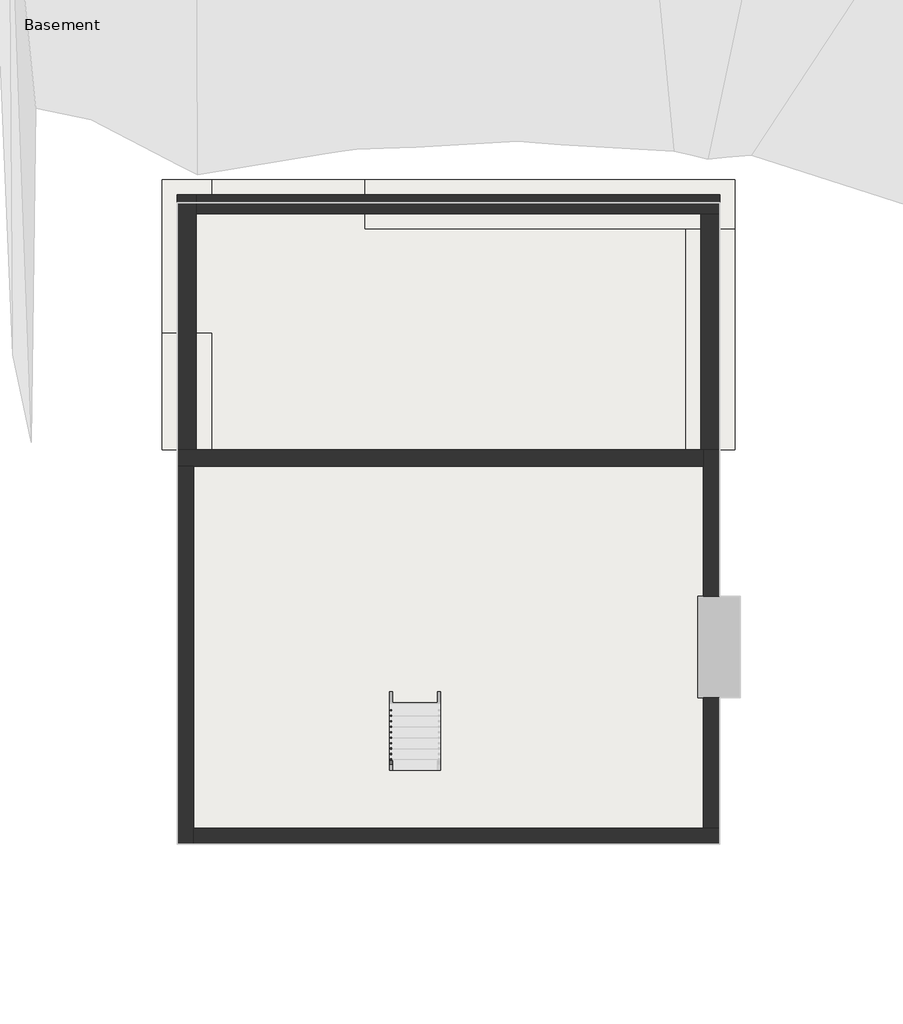
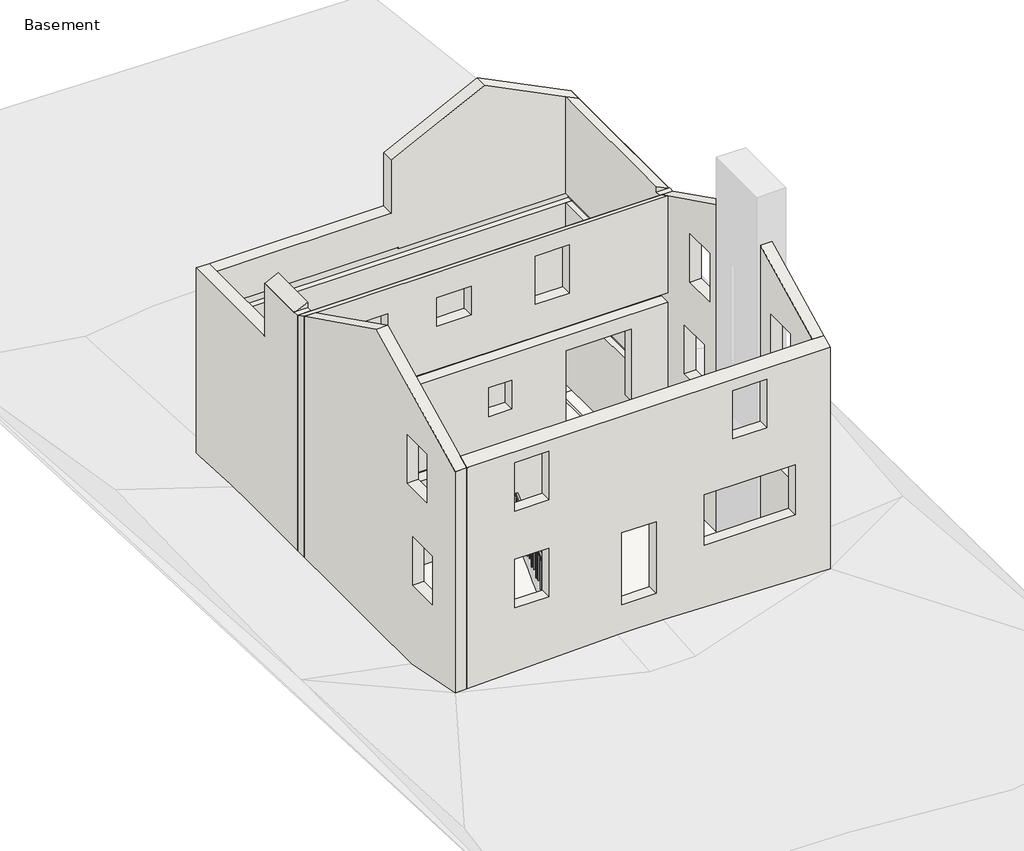
# One storey, part 1 of 2: 8 walls, 3 footings, 2 slabs, 1 railing.
"""IFC4 building model written with IfcOpenShell, lengths in millimetres."""

from ifc_helpers import new_model, si_unit, frame, origin, place, context, project, spatial, polyline, outline, extrude, faceted_brep, element, save

model = new_model("IFC4")

# Units and contexts
model_context = context("Model", 3, world=origin())
ifc_project = project(units=[si_unit("LENGTHUNIT", "METRE", prefix="MILLI")], contexts=[model_context])

# Site, building, storey
site = spatial("IfcSite", under=ifc_project)
building = spatial("IfcBuilding", under=site)
storey = spatial("IfcBuildingStorey", under=building, Name="Basement", Elevation=-2667.0)

# Footings
placement = place(None, origin())
element("IfcFooting", 1, ObjectType="Bearing Footing - 36\" x 12\"", at=placement, inside=storey, context=model_context, shape_type="Brep", body=[
    faceted_brep([(-5355.7678068, 3152.0888758, -2667.0), (-6270.1678068, 3152.0888758, -2667.0), (-6270.1678068, 3152.0888758, -2971.8), (-5355.7678068, 3152.0888758, -2971.8), (-6270.1678068, 5311.0888758, -2667.0), (-5355.7678068, 5311.0888758, -2667.0), (-5355.7678068, 5311.0888758, -2971.8), (-6270.1678068, 5311.0888758, -2971.8)], [[[0, 1, 2, 3]], [[4, 5, 6, 7]], [[0, 5, 4, 1]], [[2, 1, 4, 7]], [[3, 2, 7, 6]], [[0, 3, 6, 5]]]),
    faceted_brep([(-5355.7678068, 5311.0888758, -3124.2), (-6270.1678068, 5311.0888758, -3124.2), (-6270.1678068, 5311.0888758, -3429.0), (-5355.7678068, 5311.0888758, -3429.0), (-5355.7678068, 7243.0763758, -3124.2), (-5355.7678068, 8157.4763758, -3124.2), (-6270.1678068, 8157.4763758, -3124.2), (-6270.1678068, 8157.4763758, -3429.0), (-5355.7678068, 8157.4763758, -3429.0), (-5355.7678068, 7243.0763758, -3429.0)], [[[0, 1, 2, 3]], [[0, 4, 5, 6, 1]], [[2, 1, 6, 7]], [[3, 2, 7, 8, 9]], [[0, 3, 9, 8, 5, 4]], [[6, 5, 8, 7]]]),
])
element("IfcFooting", 2, ObjectType="Bearing Footing - 36\" x 12\"", at=placement, inside=storey, context=model_context, shape_type="Brep", body=[
    faceted_brep([(-2509.3803068, 8157.4763758, -3429.0), (-2509.3803068, 8157.4763758, -3124.2), (-2509.3803068, 7243.0763758, -3124.2), (-2509.3803068, 7243.0763758, -3429.0), (-5355.7678068, 8157.4763758, -3124.2), (-5355.7678068, 7243.0763758, -3124.2), (-5355.7678068, 8157.4763758, -3429.0), (-5355.7678068, 7243.0763758, -3429.0)], [[[0, 1, 2, 3]], [[2, 1, 4, 5]], [[1, 0, 6, 4]], [[0, 3, 7, 6]], [[3, 2, 5, 7]], [[5, 4, 6, 7]]]),
    faceted_brep([(-2509.3803068, 8157.4763758, -2667.0), (-2509.3803068, 8157.4763758, -2971.8), (-2509.3803068, 7243.0763758, -2971.8), (-2509.3803068, 7243.0763758, -2667.0), (4350.2071932, 8157.4763758, -2667.0), (3435.8071932, 7243.0763758, -2667.0), (4350.2071932, 7243.0763758, -2667.0), (4350.2071932, 8157.4763758, -2971.8), (4350.2071932, 7243.0763758, -2971.8), (3435.8071932, 7243.0763758, -2971.8)], [[[0, 1, 2, 3]], [[4, 0, 3, 5, 6]], [[1, 0, 4, 7]], [[2, 1, 7, 8, 9]], [[3, 2, 9, 8, 6, 5]], [[4, 6, 8, 7]]]),
])
element("IfcFooting", 3, ObjectType="Bearing Footing - 36\" x 12\"", at=placement, inside=storey, context=model_context, shape_type="SweptSolid", body=[
    extrude(outline(polyline([(4350.2071932, 3152.0888758), (3435.8071932, 3152.0888758), (3435.8071932, 7243.0763758), (4350.2071932, 7243.0763758), (4350.2071932, 3152.0888758)])), frame((0.0, 0.0, -2971.8), z_axis=(0.0, 0.0, 1.0), x_axis=(1.0, 0.0, 0.0)), (0.0, 0.0, 1.0), 304.8),
])

# Railing
element("IfcRailing", 4, ObjectType="Handrail - Rectangular", at=placement, inside=storey, context=model_context, shape_type="SweptSolid", body=[
    extrude(outline(polyline([(-2791.5111242, -1631.7331862), (-2791.5111242, -1562.1), (-149.9111242, 914.4), (-149.9111242, 844.7668138), (-2791.5111242, -1631.7331862)])), frame((-2052.1803068, 0.0, 0.0), z_axis=(1.0, 0.0, 0.0), x_axis=(0.0, 1.0, 0.0)), (0.0, 0.0, 1.0), 50.8),
    extrude(outline(polyline([(-241.9861242, 758.4465013), (-241.9861242, -190.5), (-261.0361242, -190.5), (-261.0361242, 740.5871263), (-241.9861242, 758.4465013)])), frame((-2036.3053068, 0.0, 0.0), z_axis=(1.0, 0.0, 0.0), x_axis=(0.0, 1.0, 0.0)), (0.0, 0.0, 1.0), 19.05),
    extrude(outline(polyline([(-343.5861242, 663.1965013), (-343.5861242, -190.5), (-362.6361242, -190.5), (-362.6361242, 645.3371263), (-343.5861242, 663.1965013)])), frame((-2036.3053068, 0.0, 0.0), z_axis=(1.0, 0.0, 0.0), x_axis=(0.0, 1.0, 0.0)), (0.0, 0.0, 1.0), 19.05),
    extrude(outline(polyline([(-445.1861242, 567.9465013), (-445.1861242, -381.0), (-464.2361242, -381.0), (-464.2361242, 550.0871263), (-445.1861242, 567.9465013)])), frame((-2036.3053068, 0.0, 0.0), z_axis=(1.0, 0.0, 0.0), x_axis=(0.0, 1.0, 0.0)), (0.0, 0.0, 1.0), 19.05),
    extrude(outline(polyline([(-546.7861242, 472.6965013), (-546.7861242, -381.0), (-565.8361242, -381.0), (-565.8361242, 454.8371263), (-546.7861242, 472.6965013)])), frame((-2036.3053068, 0.0, 0.0), z_axis=(1.0, 0.0, 0.0), x_axis=(0.0, 1.0, 0.0)), (0.0, 0.0, 1.0), 19.05),
    extrude(outline(polyline([(-648.3861242, 377.4465013), (-648.3861242, -571.5), (-667.4361242, -571.5), (-667.4361242, 359.5871263), (-648.3861242, 377.4465013)])), frame((-2036.3053068, 0.0, 0.0), z_axis=(1.0, 0.0, 0.0), x_axis=(0.0, 1.0, 0.0)), (0.0, 0.0, 1.0), 19.05),
    extrude(outline(polyline([(-749.9861242, 282.1965013), (-749.9861242, -571.5), (-769.0361242, -571.5), (-769.0361242, 264.3371263), (-749.9861242, 282.1965013)])), frame((-2036.3053068, 0.0, 0.0), z_axis=(1.0, 0.0, 0.0), x_axis=(0.0, 1.0, 0.0)), (0.0, 0.0, 1.0), 19.05),
    extrude(outline(polyline([(-851.5861242, 186.9465013), (-851.5861242, -762.0), (-870.6361242, -762.0), (-870.6361242, 169.0871263), (-851.5861242, 186.9465013)])), frame((-2036.3053068, 0.0, 0.0), z_axis=(1.0, 0.0, 0.0), x_axis=(0.0, 1.0, 0.0)), (0.0, 0.0, 1.0), 19.05),
    extrude(outline(polyline([(-953.1861242, 91.6965013), (-953.1861242, -762.0), (-972.2361242, -762.0), (-972.2361242, 73.8371263), (-953.1861242, 91.6965013)])), frame((-2036.3053068, 0.0, 0.0), z_axis=(1.0, 0.0, 0.0), x_axis=(0.0, 1.0, 0.0)), (0.0, 0.0, 1.0), 19.05),
    extrude(outline(polyline([(-1054.7861242, -3.5534987), (-1054.7861242, -952.5), (-1073.8361242, -952.5), (-1073.8361242, -21.4128737), (-1054.7861242, -3.5534987)])), frame((-2036.3053068, 0.0, 0.0), z_axis=(1.0, 0.0, 0.0), x_axis=(0.0, 1.0, 0.0)), (0.0, 0.0, 1.0), 19.05),
    extrude(outline(polyline([(-1156.3861242, -98.8034987), (-1156.3861242, -952.5), (-1175.4361242, -952.5), (-1175.4361242, -116.6628737), (-1156.3861242, -98.8034987)])), frame((-2036.3053068, 0.0, 0.0), z_axis=(1.0, 0.0, 0.0), x_axis=(0.0, 1.0, 0.0)), (0.0, 0.0, 1.0), 19.05),
    extrude(outline(polyline([(-1257.9861242, -194.0534987), (-1257.9861242, -1143.0), (-1277.0361242, -1143.0), (-1277.0361242, -211.9128737), (-1257.9861242, -194.0534987)])), frame((-2036.3053068, 0.0, 0.0), z_axis=(1.0, 0.0, 0.0), x_axis=(0.0, 1.0, 0.0)), (0.0, 0.0, 1.0), 19.05),
    extrude(outline(polyline([(-1359.5861242, -289.3034987), (-1359.5861242, -1143.0), (-1378.6361242, -1143.0), (-1378.6361242, -307.1628737), (-1359.5861242, -289.3034987)])), frame((-2036.3053068, 0.0, 0.0), z_axis=(1.0, 0.0, 0.0), x_axis=(0.0, 1.0, 0.0)), (0.0, 0.0, 1.0), 19.05),
    extrude(outline(polyline([(-1461.1861242, -384.5534987), (-1461.1861242, -1333.5), (-1480.2361242, -1333.5), (-1480.2361242, -402.4128737), (-1461.1861242, -384.5534987)])), frame((-2036.3053068, 0.0, 0.0), z_axis=(1.0, 0.0, 0.0), x_axis=(0.0, 1.0, 0.0)), (0.0, 0.0, 1.0), 19.05),
    extrude(outline(polyline([(-1562.7861242, -479.8034987), (-1562.7861242, -1333.5), (-1581.8361242, -1333.5), (-1581.8361242, -497.6628737), (-1562.7861242, -479.8034987)])), frame((-2036.3053068, 0.0, 0.0), z_axis=(1.0, 0.0, 0.0), x_axis=(0.0, 1.0, 0.0)), (0.0, 0.0, 1.0), 19.05),
    extrude(outline(polyline([(-1664.3861242, -575.0534987), (-1664.3861242, -1524.0), (-1683.4361242, -1524.0), (-1683.4361242, -592.9128737), (-1664.3861242, -575.0534987)])), frame((-2036.3053068, 0.0, 0.0), z_axis=(1.0, 0.0, 0.0), x_axis=(0.0, 1.0, 0.0)), (0.0, 0.0, 1.0), 19.05),
    extrude(outline(polyline([(-1765.9861242, -670.3034987), (-1765.9861242, -1524.0), (-1785.0361242, -1524.0), (-1785.0361242, -688.1628737), (-1765.9861242, -670.3034987)])), frame((-2036.3053068, 0.0, 0.0), z_axis=(1.0, 0.0, 0.0), x_axis=(0.0, 1.0, 0.0)), (0.0, 0.0, 1.0), 19.05),
    extrude(outline(polyline([(-1867.5861242, -765.5534987), (-1867.5861242, -1714.5), (-1886.6361242, -1714.5), (-1886.6361242, -783.4128737), (-1867.5861242, -765.5534987)])), frame((-2036.3053068, 0.0, 0.0), z_axis=(1.0, 0.0, 0.0), x_axis=(0.0, 1.0, 0.0)), (0.0, 0.0, 1.0), 19.05),
    extrude(outline(polyline([(-1969.1861242, -860.8034987), (-1969.1861242, -1714.5), (-1988.2361242, -1714.5), (-1988.2361242, -878.6628737), (-1969.1861242, -860.8034987)])), frame((-2036.3053068, 0.0, 0.0), z_axis=(1.0, 0.0, 0.0), x_axis=(0.0, 1.0, 0.0)), (0.0, 0.0, 1.0), 19.05),
    extrude(outline(polyline([(-2070.7861242, -956.0534987), (-2070.7861242, -1905.0), (-2089.8361242, -1905.0), (-2089.8361242, -973.9128737), (-2070.7861242, -956.0534987)])), frame((-2036.3053068, 0.0, 0.0), z_axis=(1.0, 0.0, 0.0), x_axis=(0.0, 1.0, 0.0)), (0.0, 0.0, 1.0), 19.05),
    extrude(outline(polyline([(-2172.3861242, -1051.3034987), (-2172.3861242, -1905.0), (-2191.4361242, -1905.0), (-2191.4361242, -1069.1628737), (-2172.3861242, -1051.3034987)])), frame((-2036.3053068, 0.0, 0.0), z_axis=(1.0, 0.0, 0.0), x_axis=(0.0, 1.0, 0.0)), (0.0, 0.0, 1.0), 19.05),
    extrude(outline(polyline([(-2273.9861242, -1146.5534987), (-2273.9861242, -2095.5), (-2293.0361242, -2095.5), (-2293.0361242, -1164.4128737), (-2273.9861242, -1146.5534987)])), frame((-2036.3053068, 0.0, 0.0), z_axis=(1.0, 0.0, 0.0), x_axis=(0.0, 1.0, 0.0)), (0.0, 0.0, 1.0), 19.05),
    extrude(outline(polyline([(-2375.5861242, -1241.8034987), (-2375.5861242, -2095.5), (-2394.6361242, -2095.5), (-2394.6361242, -1259.6628737), (-2375.5861242, -1241.8034987)])), frame((-2036.3053068, 0.0, 0.0), z_axis=(1.0, 0.0, 0.0), x_axis=(0.0, 1.0, 0.0)), (0.0, 0.0, 1.0), 19.05),
    extrude(outline(polyline([(-2477.1861242, -1337.0534987), (-2477.1861242, -2286.0), (-2496.2361242, -2286.0), (-2496.2361242, -1354.9128737), (-2477.1861242, -1337.0534987)])), frame((-2036.3053068, 0.0, 0.0), z_axis=(1.0, 0.0, 0.0), x_axis=(0.0, 1.0, 0.0)), (0.0, 0.0, 1.0), 19.05),
    extrude(outline(polyline([(-2578.7861242, -1432.3034987), (-2578.7861242, -2286.0), (-2597.8361242, -2286.0), (-2597.8361242, -1450.1628737), (-2578.7861242, -1432.3034987)])), frame((-2036.3053068, 0.0, 0.0), z_axis=(1.0, 0.0, 0.0), x_axis=(0.0, 1.0, 0.0)), (0.0, 0.0, 1.0), 19.05),
    extrude(outline(polyline([(-2680.3861242, -1527.5534987), (-2680.3861242, -2476.5), (-2699.4361242, -2476.5), (-2699.4361242, -1545.4128737), (-2680.3861242, -1527.5534987)])), frame((-2036.3053068, 0.0, 0.0), z_axis=(1.0, 0.0, 0.0), x_axis=(0.0, 1.0, 0.0)), (0.0, 0.0, 1.0), 19.05),
    extrude(outline(polyline([(-149.9111242, 844.7668138), (-149.9111242, -190.5), (-168.9611242, -190.5), (-168.9611242, 826.9074388), (-149.9111242, 844.7668138)])), frame((-2036.3053068, 0.0, 0.0), z_axis=(1.0, 0.0, 0.0), x_axis=(0.0, 1.0, 0.0)), (0.0, 0.0, 1.0), 19.05),
    extrude(outline(polyline([(-2772.4611242, -1613.8738112), (-2772.4611242, -2476.5), (-2791.5111242, -2476.5), (-2791.5111242, -1631.7331862), (-2772.4611242, -1613.8738112)])), frame((-2036.3053068, 0.0, 0.0), z_axis=(1.0, 0.0, 0.0), x_axis=(0.0, 1.0, 0.0)), (0.0, 0.0, 1.0), 19.05),
])

# Slabs
element("IfcSlab", 5, ObjectType="Pad 1", at=placement, inside=storey, context=model_context, shape_type="SweptSolid", body=[
    extrude(outline(polyline([(4069.2196932, 434.2888758), (4450.2196932, 434.2888758), (4450.2196932, -1445.3111242), (4069.2196932, -1445.3111242), (4069.2196932, -4163.1111242), (-5989.1803068, -4163.1111242), (-5989.1803068, 3152.0888758), (4069.2196932, 3152.0888758), (4069.2196932, 434.2888758)])), frame((0.0, 0.0, -3073.4), z_axis=(0.0, 0.0, 1.0), x_axis=(1.0, 0.0, 0.0)), (0.0, 0.0, 1.0), 304.8),
])
element("IfcSlab", 6, ObjectType="Pad 1", at=placement, inside=storey, context=model_context, shape_type="SweptSolid", body=[
    extrude(outline(polyline([(-5989.1803068, 7724.0888758), (4069.2196932, 7724.0888758), (4069.2196932, 3152.0888758), (-5989.1803068, 3152.0888758), (-5989.1803068, 7724.0888758)])), frame((0.0, 0.0, -3073.4), z_axis=(0.0, 0.0, 1.0), x_axis=(1.0, 0.0, 0.0)), (0.0, 0.0, 1.0), 304.8),
])

# Walls
element("IfcWall", 7, ObjectType="Exterior - Brick on Mtl. Stud", at=placement, inside=storey, context=model_context, shape_type="Brep", body=[
    faceted_brep([(-5636.7553068, 3152.0888758, -2667.0), (-5636.7553068, 5311.0888758, -2667.0), (-5636.7553068, 5311.0888758, -3124.2), (-5636.7553068, 7524.0638758, -3124.2), (-5636.7553068, 7876.4888758, -3124.2), (-5636.7553068, 7876.4888758, 3810.0), (-5636.7553068, 7524.0638758, 3810.0), (-5636.7553068, 4676.0888758, 3810.0), (-5636.7553068, 4676.0888758, 5486.4), (-5636.7553068, 4323.6638758, 5486.4), (-5636.7553068, 3304.4888758, 5486.4), (-5636.7553068, 3304.4888758, 5336.1342644), (-5636.7553068, 3152.0888758, 5336.1342644), (-5636.7553068, 3152.0888758, 2743.2), (-5636.7553068, 4323.6638758, 2743.2), (-5636.7553068, 4488.7638758, 2743.2), (-5636.7553068, 4488.7638758, 2781.3), (-5636.7553068, 7524.0638758, 2781.3), (-5636.7553068, 7689.1638758, 2781.3), (-5636.7553068, 7689.1638758, 2470.15), (-5636.7553068, 7524.0638758, 2470.15), (-5636.7553068, 3152.0888758, 2470.15), (-5636.7553068, 3152.0888758, 0.0), (-5636.7553068, 7524.0638758, 0.0), (-5636.7553068, 7689.1638758, 0.0), (-5636.7553068, 7689.1638758, -273.05), (-5636.7553068, 7524.0638758, -273.05), (-5636.7553068, 3152.0888758, -273.05), (-5989.1803068, 5311.0888758, -2667.0), (-5989.1803068, 3152.0888758, -2667.0), (-5989.1803068, 3152.0888758, 5336.1342644), (-5989.1803068, 3304.4888758, 5336.1342644), (-5989.1803068, 3304.4888758, 5312.3217644), (-5989.1803068, 4676.0888758, 5312.3217644), (-5989.1803068, 4676.0888758, 3810.0), (-5989.1803068, 7876.4888758, 3810.0), (-5989.1803068, 7876.4888758, -3124.2), (-5989.1803068, 5311.0888758, -3124.2), (-5801.8553068, 3152.0888758, -273.05), (-5801.8553068, 3152.0888758, 0.0), (-5801.8553068, 3152.0888758, 2470.15), (-5801.8553068, 3152.0888758, 2743.2), (-5984.911778, 4676.0888758, 5312.3217644), (-5937.286778, 3304.4888758, 5336.1342644), (-5984.911778, 3304.4888758, 5312.3217644), (-5801.8553068, 7689.1638758, -273.05), (-5801.8553068, 7689.1638758, 0.0), (-5801.8553068, 7689.1638758, 2470.15), (-5801.8553068, 4488.7638758, 2470.15), (-5801.8553068, 4488.7638758, 2743.2), (-5801.8553068, 7689.1638758, 2781.3), (-5801.8553068, 4488.7638758, 2781.3)], [[[0, 1, 2, 3, 4, 5, 6, 7, 8, 9, 10, 11, 12, 13, 14, 15, 16, 17, 18, 19, 20, 21, 22, 23, 24, 25, 26, 27]], [[28, 29, 30, 31, 32, 33, 34, 35, 36, 37]], [[5, 4, 36, 35]], [[1, 0, 29, 28]], [[2, 1, 28, 37]], [[4, 3, 2, 37, 36]], [[30, 29, 0, 27, 38, 39, 22, 21, 40, 41, 13, 12]], [[7, 6, 5, 35, 34]], [[8, 7, 34, 33, 42]], [[32, 31, 43, 44]], [[10, 9, 8, 42, 44, 43]], [[33, 32, 44, 42]], [[12, 11, 43, 31, 30]], [[11, 10, 43]], [[45, 38, 27, 26, 25]], [[46, 24, 23, 22, 39]], [[46, 45, 25, 24]], [[45, 46, 39, 38]], [[40, 21, 20, 19, 47, 48]], [[41, 49, 15, 14, 13]], [[40, 48, 47, 50, 51, 49, 41]], [[51, 50, 18, 17, 16]], [[50, 47, 19, 18]], [[49, 51, 16, 15]]]),
])
element("IfcWall", 8, ObjectType="Exterior - Brick on Mtl. Stud", at=placement, inside=storey, context=model_context, shape_type="Brep", body=[
    faceted_brep([(-2509.3803068, 7524.0638758, -2667.0), (3716.7946932, 7524.0638758, -2667.0), (4069.2196932, 7524.0638758, -2667.0), (4069.2196932, 7524.0638758, 5312.3217644), (4064.9511643, 7524.0638758, 5312.3217644), (3716.7946932, 7524.0638758, 5486.4), (1554.6196932, 7524.0638758, 6567.4875), (-607.5553068, 7524.0638758, 5486.4), (-955.711778, 7524.0638758, 5312.3217644), (-959.9803068, 7524.0638758, 5312.3217644), (-959.9803068, 7524.0638758, 3810.0), (-5636.7553068, 7524.0638758, 3810.0), (-5636.7553068, 7524.0638758, 2781.3), (-772.6553068, 7524.0638758, 2781.3), (-772.6553068, 7524.0638758, 2743.2), (-607.5553068, 7524.0638758, 2743.2), (3716.7946932, 7524.0638758, 2743.2), (3881.8946932, 7524.0638758, 2743.2), (3881.8946932, 7524.0638758, 2470.15), (3716.7946932, 7524.0638758, 2470.15), (-5636.7553068, 7524.0638758, 2470.15), (-5636.7553068, 7524.0638758, 0.0), (3716.7946932, 7524.0638758, 0.0), (3881.8946932, 7524.0638758, 0.0), (3881.8946932, 7524.0638758, -273.05), (3716.7946932, 7524.0638758, -273.05), (-5636.7553068, 7524.0638758, -273.05), (-5636.7553068, 7524.0638758, -3124.2), (-2509.3803068, 7524.0638758, -3124.2), (4069.2196932, 7876.4888758, -2667.0), (-2509.3803068, 7876.4888758, -2667.0), (-2509.3803068, 7876.4888758, -3124.2), (-5636.7553068, 7876.4888758, -3124.2), (-5636.7553068, 7876.4888758, 3810.0), (-959.9803068, 7876.4888758, 3810.0), (-959.9803068, 7876.4888758, 5312.3217644), (-955.711778, 7876.4888758, 5312.3217644), (1554.6196932, 7876.4888758, 6567.4875), (4064.9511643, 7876.4888758, 5312.3217644), (4069.2196932, 7876.4888758, 5312.3217644), (-5636.7553068, 7689.1638758, -273.05), (-5636.7553068, 7689.1638758, 0.0), (-5636.7553068, 7689.1638758, 2470.15), (-5636.7553068, 7689.1638758, 2781.3), (3881.8946932, 7689.1638758, -273.05), (3881.8946932, 7689.1638758, 0.0), (3881.8946932, 7689.1638758, 2470.15), (-772.6553068, 7689.1638758, 2470.15), (-772.6553068, 7689.1638758, 2743.2), (3881.8946932, 7689.1638758, 2743.2), (-772.6553068, 7689.1638758, 2781.3)], [[[0, 1, 2, 3, 4, 5, 6, 7, 8, 9, 10, 11, 12, 13, 14, 15, 16, 17, 18, 19, 20, 21, 22, 23, 24, 25, 26, 27, 28]], [[29, 30, 31, 32, 33, 34, 35, 36, 37, 38, 39]], [[33, 32, 27, 26, 40, 41, 21, 20, 42, 43, 12, 11]], [[3, 2, 29, 39]], [[2, 1, 0, 30, 29]], [[28, 27, 32, 31]], [[0, 28, 31, 30]], [[11, 10, 34, 33]], [[10, 9, 35, 34]], [[35, 9, 8, 36]], [[8, 7, 6, 37, 36]], [[6, 5, 4, 38, 37]], [[3, 39, 38, 4]], [[24, 44, 40, 26, 25]], [[41, 45, 23, 22, 21]], [[44, 45, 41, 40]], [[45, 44, 24, 23]], [[42, 20, 19, 18, 46, 47]], [[48, 49, 17, 16, 15, 14]], [[42, 47, 46, 49, 48, 50, 43]], [[49, 46, 18, 17]], [[43, 50, 13, 12]], [[50, 48, 14, 13]]]),
])
element("IfcWall", 9, ObjectType="Exterior - Brick on Mtl. Stud", at=placement, inside=storey, context=model_context, shape_type="Brep", body=[
    faceted_brep([(3716.7946932, 7524.0638758, -2667.0), (3716.7946932, 3152.0888758, -2667.0), (3716.7946932, 3152.0888758, -273.05), (3716.7946932, 7524.0638758, -273.05), (3716.7946932, 3304.4888758, 5336.1342644), (3716.7946932, 3304.4888758, 5486.4), (3716.7946932, 7524.0638758, 5486.4), (3716.7946932, 7524.0638758, 2743.2), (3716.7946932, 3152.0888758, 2743.2), (3716.7946932, 3152.0888758, 5336.1342644), (3716.7946932, 7524.0638758, 0.0), (3716.7946932, 3152.0888758, 0.0), (3716.7946932, 3152.0888758, 2470.15), (3716.7946932, 7524.0638758, 2470.15), (4069.2196932, 3152.0888758, -2667.0), (4069.2196932, 7524.0638758, -2667.0), (4069.2196932, 7524.0638758, 5312.3217644), (4069.2196932, 3304.4888758, 5312.3217644), (4069.2196932, 3304.4888758, 5336.1342644), (4069.2196932, 3152.0888758, 5336.1342644), (3881.8946932, 7524.0638758, -273.05), (3881.8946932, 7524.0638758, 0.0), (3881.8946932, 7524.0638758, 2470.15), (3881.8946932, 7524.0638758, 2743.2), (4064.9511643, 7524.0638758, 5312.3217644), (3881.8946932, 3152.0888758, 2743.2), (3881.8946932, 3152.0888758, 2470.15), (3881.8946932, 3152.0888758, 0.0), (3881.8946932, 3152.0888758, -273.05), (4064.9511643, 3304.4888758, 5312.3217644), (4017.3261643, 3304.4888758, 5336.1342644)], [[[0, 1, 2, 3]], [[4, 5, 6, 7, 8, 9]], [[10, 11, 12, 13]], [[14, 15, 16, 17, 18, 19]], [[1, 0, 15, 14]], [[16, 15, 0, 3, 20, 21, 10, 13, 22, 23, 7, 6, 24]], [[1, 14, 19, 9, 8, 25, 26, 12, 11, 27, 28, 2]], [[18, 17, 29, 30]], [[4, 9, 19, 18, 30]], [[6, 5, 30, 29, 24]], [[17, 16, 24, 29]], [[5, 4, 30]], [[28, 20, 3, 2]], [[21, 27, 11, 10]], [[20, 28, 27, 21]], [[26, 22, 13, 12]], [[23, 25, 8, 7]], [[22, 26, 25, 23]]]),
])
element("IfcWall", 10, ObjectType="Generic - 12\"", at=placement, inside=storey, context=model_context, shape_type="Brep", body=[
    faceted_brep([(-5989.1803068, 2847.2888758, -2667.0), (-5684.3803068, 2847.2888758, -2667.0), (3764.4196932, 2847.2888758, -2667.0), (3764.4196932, 2847.2888758, -273.05), (-5801.8553068, 2847.2888758, -273.05), (-5801.8553068, 2847.2888758, 0.0), (-5023.9803068, 2847.2888758, 0.0), (-5023.9803068, 2847.2888758, 2032.0), (-4160.3803068, 2847.2888758, 2032.0), (-4160.3803068, 2847.2888758, 0.0), (-1518.7803068, 2847.2888758, 0.0), (-1391.7803068, 2847.2888758, 0.0), (-70.9803068, 2847.2888758, 0.0), (56.0196932, 2847.2888758, 0.0), (1021.2196932, 2847.2888758, 0.0), (1021.2196932, 2847.2888758, 2057.4), (2799.2196932, 2847.2888758, 2057.4), (2799.2196932, 2847.2888758, 0.0), (3764.4196932, 2847.2888758, 0.0), (3764.4196932, 2847.2888758, 2470.15), (-5801.8553068, 2847.2888758, 2470.15), (-5801.8553068, 2847.2888758, 2743.2), (-3296.7803068, 2847.2888758, 2743.2), (-3169.7803068, 2847.2888758, 2743.2), (-807.5803068, 2847.2888758, 2743.2), (-680.5803068, 2847.2888758, 2743.2), (-70.9803068, 2847.2888758, 2743.2), (56.0196932, 2847.2888758, 2743.2), (3764.4196932, 2847.2888758, 2743.2), (3764.4196932, 2847.2888758, 5486.4), (-5684.3803068, 2847.2888758, 5486.4), (-5989.1803068, 2847.2888758, 5486.4), (-1036.1803068, 2847.2888758, 914.4), (-1036.1803068, 2847.2888758, 1727.2), (-426.5803068, 2847.2888758, 1727.2), (-426.5803068, 2847.2888758, 914.4), (-3919.0803068, 2847.2888758, 914.4), (-3919.0803068, 2847.2888758, 1727.2), (-3004.6803068, 2847.2888758, 1727.2), (-3004.6803068, 2847.2888758, 914.4), (208.4196932, 2847.2888758, 3657.6), (208.4196932, 2847.2888758, 5029.2), (1122.8196932, 2847.2888758, 5029.2), (1122.8196932, 2847.2888758, 3657.6), (-2433.1803068, 2847.2888758, 3962.4), (-2433.1803068, 2847.2888758, 4775.2), (-1518.7803068, 2847.2888758, 4775.2), (-1518.7803068, 2847.2888758, 3962.4), (-4668.3803068, 2847.2888758, 3962.4), (-4668.3803068, 2847.2888758, 4775.2), (-3753.9803068, 2847.2888758, 4775.2), (-3753.9803068, 2847.2888758, 3962.4), (3764.4196932, 3152.0888758, -2667.0), (-5989.1803068, 3152.0888758, -2667.0), (-5989.1803068, 3152.0888758, 5336.1342644), (3764.4196932, 3152.0888758, 5336.1342644), (3764.4196932, 3152.0888758, 2743.2), (-5801.8553068, 3152.0888758, 2743.2), (-5801.8553068, 3152.0888758, 2470.15), (3764.4196932, 3152.0888758, 2470.15), (3764.4196932, 3152.0888758, 0.0), (2799.2196932, 3152.0888758, 0.0), (2799.2196932, 3152.0888758, 2057.4), (1021.2196932, 3152.0888758, 2057.4), (1021.2196932, 3152.0888758, 0.0), (-4160.3803068, 3152.0888758, 0.0), (-4160.3803068, 3152.0888758, 2032.0), (-5023.9803068, 3152.0888758, 2032.0), (-5023.9803068, 3152.0888758, 0.0), (-5801.8553068, 3152.0888758, 0.0), (-5801.8553068, 3152.0888758, -273.05), (3764.4196932, 3152.0888758, -273.05), (-1036.1803068, 3152.0888758, 1727.2), (-1036.1803068, 3152.0888758, 914.4), (-426.5803068, 3152.0888758, 914.4), (-426.5803068, 3152.0888758, 1727.2), (-3919.0803068, 3152.0888758, 1727.2), (-3919.0803068, 3152.0888758, 914.4), (-3004.6803068, 3152.0888758, 914.4), (-3004.6803068, 3152.0888758, 1727.2), (208.4196932, 3152.0888758, 5029.2), (208.4196932, 3152.0888758, 3657.6), (1122.8196932, 3152.0888758, 3657.6), (1122.8196932, 3152.0888758, 5029.2), (-2433.1803068, 3152.0888758, 4775.2), (-2433.1803068, 3152.0888758, 3962.4), (-1518.7803068, 3152.0888758, 3962.4), (-1518.7803068, 3152.0888758, 4775.2), (-4668.3803068, 3152.0888758, 4775.2), (-4668.3803068, 3152.0888758, 3962.4), (-3753.9803068, 3152.0888758, 3962.4), (-3753.9803068, 3152.0888758, 4775.2), (-5989.1803068, 3147.820347, 5336.1342644), (3764.4196932, 3147.820347, 5336.1342644)], [[[0, 1, 2, 3, 4, 5, 6, 7, 8, 9, 10, 11, 12, 13, 14, 15, 16, 17, 18, 19, 20, 21, 22, 23, 24, 25, 26, 27, 28, 29, 30, 31], [32, 33, 34, 35], [36, 37, 38, 39], [40, 41, 42, 43], [44, 45, 46, 47], [48, 49, 50, 51]], [[52, 53, 54, 55, 56, 57, 58, 59, 60, 61, 62, 63, 64, 65, 66, 67, 68, 69, 70, 71], [72, 73, 74, 75], [76, 77, 78, 79], [80, 81, 82, 83], [84, 85, 86, 87], [88, 89, 90, 91]], [[2, 1, 0, 53, 52]], [[0, 31, 92, 54, 53]], [[2, 52, 71, 3]], [[93, 29, 28, 56, 55]], [[18, 60, 59, 19]], [[63, 15, 14, 64]], [[15, 63, 62, 16]], [[16, 62, 61, 17]], [[7, 6, 68, 67]], [[8, 7, 67, 66]], [[9, 8, 66, 65]], [[73, 72, 33, 32]], [[74, 73, 32, 35]], [[75, 74, 35, 34]], [[72, 75, 34, 33]], [[77, 76, 37, 36]], [[78, 77, 36, 39]], [[79, 78, 39, 38]], [[76, 79, 38, 37]], [[41, 40, 81, 80]], [[40, 43, 82, 81]], [[43, 42, 83, 82]], [[42, 41, 80, 83]], [[45, 44, 85, 84]], [[44, 47, 86, 85]], [[47, 46, 87, 86]], [[46, 45, 84, 87]], [[49, 48, 89, 88]], [[48, 51, 90, 89]], [[51, 50, 91, 90]], [[50, 49, 88, 91]], [[31, 30, 29, 93, 92]], [[55, 54, 92, 93]], [[70, 4, 3, 71]], [[14, 13, 12, 11, 10, 9, 65, 64]], [[18, 17, 61, 60]], [[5, 69, 68, 6]], [[4, 70, 69, 5]], [[58, 20, 19, 59]], [[21, 57, 56, 28, 27, 26, 25, 24, 23, 22]], [[20, 58, 57, 21]]]),
])
element("IfcWall", 11, ObjectType="Generic - 12\"", at=placement, inside=storey, context=model_context, shape_type="Brep", body=[
    faceted_brep([(-5684.3803068, -4163.1111242, -2667.0), (-5684.3803068, -3858.3111242, -2667.0), (-5684.3803068, 2847.2888758, -2667.0), (-5684.3803068, 2847.2888758, 5486.4), (-5684.3803068, -505.5111242, 7162.8), (-5684.3803068, -3858.3111242, 5486.4), (-5684.3803068, -4158.8425953, 5336.1342644), (-5684.3803068, -4163.1111242, 5336.1342644), (-5684.3803068, -3096.3111242, 2286.0), (-5684.3803068, -2181.9111242, 2286.0), (-5684.3803068, -2181.9111242, 914.4), (-5684.3803068, -3096.3111242, 914.4), (-5684.3803068, -2842.3111242, 3657.6), (-5684.3803068, -2842.3111242, 5029.2), (-5684.3803068, -1927.9111242, 5029.2), (-5684.3803068, -1927.9111242, 3657.6), (-5989.1803068, 2847.2888758, -2667.0), (-5989.1803068, -4163.1111242, -2667.0), (-5989.1803068, -4163.1111242, 5336.1342644), (-5989.1803068, -4158.8425953, 5336.1342644), (-5989.1803068, -505.5111242, 7162.8), (-5989.1803068, 2847.2888758, 5486.4), (-5989.1803068, -3096.3111242, 2286.0), (-5989.1803068, -3096.3111242, 914.4), (-5989.1803068, -2181.9111242, 914.4), (-5989.1803068, -2181.9111242, 2286.0), (-5989.1803068, -2842.3111242, 5029.2), (-5989.1803068, -2842.3111242, 3657.6), (-5989.1803068, -1927.9111242, 3657.6), (-5989.1803068, -1927.9111242, 5029.2)], [[[0, 1, 2, 3, 4, 5, 6, 7], [8, 9, 10, 11], [12, 13, 14, 15]], [[16, 17, 18, 19, 20, 21], [22, 23, 24, 25], [26, 27, 28, 29]], [[2, 1, 0, 17, 16]], [[0, 7, 18, 17]], [[3, 2, 16, 21]], [[23, 22, 8, 11]], [[24, 23, 11, 10]], [[25, 24, 10, 9]], [[22, 25, 9, 8]], [[26, 13, 12, 27]], [[27, 12, 15, 28]], [[28, 15, 14, 29]], [[13, 26, 29, 14]], [[3, 21, 20, 4]], [[18, 7, 6, 19]], [[6, 5, 4, 20, 19]]]),
])
element("IfcWall", 12, ObjectType="Generic - 12\"", at=placement, inside=storey, context=model_context, shape_type="Brep", body=[
    faceted_brep([(4069.2196932, -3858.3111242, -2667.0), (3764.4196932, -3858.3111242, -2667.0), (-5684.3803068, -3858.3111242, -2667.0), (-5684.3803068, -3858.3111242, 5486.4), (3764.4196932, -3858.3111242, 5486.4), (4069.2196932, -3858.3111242, 5486.4), (-604.3803068, -3858.3111242, 0.0), (-604.3803068, -3858.3111242, 2032.0), (-1518.7803068, -3858.3111242, 2032.0), (-1518.7803068, -3858.3111242, 0.0), (-3474.5803068, -3858.3111242, 2286.0), (-4388.9803068, -3858.3111242, 2286.0), (-4388.9803068, -3858.3111242, 914.4), (-3474.5803068, -3858.3111242, 914.4), (2367.4196932, -3858.3111242, 3657.6), (2367.4196932, -3858.3111242, 5029.2), (1453.0196932, -3858.3111242, 5029.2), (1453.0196932, -3858.3111242, 3657.6), (-3474.5803068, -3858.3111242, 3657.6), (-3474.5803068, -3858.3111242, 5029.2), (-4388.9803068, -3858.3111242, 5029.2), (-4388.9803068, -3858.3111242, 3657.6), (3129.4196932, -3858.3111242, 2336.8), (691.0196932, -3858.3111242, 2336.8), (691.0196932, -3858.3111242, 914.4), (3129.4196932, -3858.3111242, 914.4), (-5684.3803068, -4163.1111242, -2667.0), (4069.2196932, -4163.1111242, -2667.0), (4069.2196932, -4163.1111242, 5336.1342644), (-5684.3803068, -4163.1111242, 5336.1342644), (-604.3803068, -4163.1111242, 0.0), (-1518.7803068, -4163.1111242, 0.0), (-1518.7803068, -4163.1111242, 2032.0), (-604.3803068, -4163.1111242, 2032.0), (-3474.5803068, -4163.1111242, 2286.0), (-3474.5803068, -4163.1111242, 914.4), (-4388.9803068, -4163.1111242, 914.4), (-4388.9803068, -4163.1111242, 2286.0), (2367.4196932, -4163.1111242, 5029.2), (2367.4196932, -4163.1111242, 3657.6), (1453.0196932, -4163.1111242, 3657.6), (1453.0196932, -4163.1111242, 5029.2), (-3474.5803068, -4163.1111242, 5029.2), (-3474.5803068, -4163.1111242, 3657.6), (-4388.9803068, -4163.1111242, 3657.6), (-4388.9803068, -4163.1111242, 5029.2), (3129.4196932, -4163.1111242, 914.4), (691.0196932, -4163.1111242, 914.4), (691.0196932, -4163.1111242, 2336.8), (3129.4196932, -4163.1111242, 2336.8), (4069.2196932, -4158.8425953, 5336.1342644), (-5684.3803068, -4158.8425953, 5336.1342644)], [[[0, 1, 2, 3, 4, 5], [6, 7, 8, 9], [10, 11, 12, 13], [14, 15, 16, 17], [18, 19, 20, 21], [22, 23, 24, 25]], [[26, 27, 28, 29], [30, 31, 32, 33], [34, 35, 36, 37], [38, 39, 40, 41], [42, 43, 44, 45], [46, 47, 48, 49]], [[2, 1, 0, 27, 26]], [[0, 5, 50, 28, 27]], [[3, 2, 26, 29, 51]], [[31, 30, 6, 9]], [[32, 31, 9, 8]], [[33, 32, 8, 7]], [[30, 33, 7, 6]], [[35, 34, 10, 13]], [[36, 35, 13, 12]], [[37, 36, 12, 11]], [[34, 37, 11, 10]], [[24, 47, 46, 25]], [[48, 23, 22, 49]], [[23, 48, 47, 24]], [[25, 46, 49, 22]], [[15, 14, 39, 38]], [[14, 17, 40, 39]], [[17, 16, 41, 40]], [[16, 15, 38, 41]], [[19, 18, 43, 42]], [[18, 21, 44, 43]], [[21, 20, 45, 44]], [[20, 19, 42, 45]], [[5, 4, 3, 51, 50]], [[29, 28, 50, 51]]]),
])
element("IfcWall", 13, ObjectType="Generic - 12\"", at=placement, inside=storey, context=model_context, shape_type="Brep", body=[
    faceted_brep([(3764.4196932, 3152.0888758, -2667.0), (3764.4196932, 2847.2888758, -2667.0), (3764.4196932, 434.2888758, -2667.0), (3764.4196932, 434.2888758, 6692.9), (3764.4196932, 2847.2888758, 5486.4), (3764.4196932, 3147.820347, 5336.1342644), (3764.4196932, 3152.0888758, 5336.1342644), (3764.4196932, 2085.2888758, 2286.0), (3764.4196932, 1170.8888758, 2286.0), (3764.4196932, 1170.8888758, 914.4), (3764.4196932, 2085.2888758, 914.4), (3764.4196932, 1831.2888758, 3657.6), (3764.4196932, 1831.2888758, 5029.2), (3764.4196932, 916.8888758, 5029.2), (3764.4196932, 916.8888758, 3657.6), (4069.2196932, 434.2888758, -2667.0), (4069.2196932, 3152.0888758, -2667.0), (4069.2196932, 3152.0888758, 5336.1342644), (4069.2196932, 3147.820347, 5336.1342644), (4069.2196932, 434.2888758, 6692.9), (4069.2196932, 2085.2888758, 2286.0), (4069.2196932, 2085.2888758, 914.4), (4069.2196932, 1170.8888758, 914.4), (4069.2196932, 1170.8888758, 2286.0), (4069.2196932, 1831.2888758, 5029.2), (4069.2196932, 1831.2888758, 3657.6), (4069.2196932, 916.8888758, 3657.6), (4069.2196932, 916.8888758, 5029.2)], [[[0, 1, 2, 3, 4, 5, 6], [7, 8, 9, 10], [11, 12, 13, 14]], [[15, 16, 17, 18, 19], [20, 21, 22, 23], [24, 25, 26, 27]], [[2, 1, 0, 16, 15]], [[3, 2, 15, 19]], [[0, 6, 17, 16]], [[21, 20, 7, 10]], [[22, 21, 10, 9]], [[23, 22, 9, 8]], [[20, 23, 8, 7]], [[24, 12, 11, 25]], [[25, 11, 14, 26]], [[26, 14, 13, 27]], [[12, 24, 27, 13]], [[17, 6, 5, 18]], [[3, 19, 18, 5, 4]]]),
])
element("IfcWall", 14, ObjectType="Generic - 12\"", at=placement, inside=storey, context=model_context, shape_type="SweptSolid", body=[
    extrude(outline(polyline([(-1445.3111242, -2667.0), (-3858.3111242, -2667.0), (-3858.3111242, 5486.4), (-1445.3111242, 6692.9), (-1445.3111242, -2667.0)]), holes=[polyline([(-2181.9111242, 2286.0), (-3096.3111242, 2286.0), (-3096.3111242, 914.4), (-2181.9111242, 914.4), (-2181.9111242, 2286.0)]), polyline([(-1927.9111242, 3657.6), (-1927.9111242, 5029.2), (-2842.3111242, 5029.2), (-2842.3111242, 3657.6), (-1927.9111242, 3657.6)])]), frame((3764.4196932, 0.0, 0.0), z_axis=(1.0, 0.0, 0.0), x_axis=(0.0, 1.0, 0.0)), (0.0, 0.0, 1.0), 304.8),
])

save(model, "model.ifc")

# Revit data of these elements
# Project information
#   Organization Name = "G3B Press"
#   Organization Description = "Paul F. Aubin Cosulting Services, Inc."
#   Building Name = "Revit Essentials for Architecture"
#   Author = "Paul F. Aubin"
#   Author Website = "https://www.paulaubin.com"
#   Copyright = "Copyright © 2020 Paul F Aubin, all rights reserved"
#   Project Issue Date = "8/1/2020"
#   Project Status = "Design Development"
#   Client Name = "Floors and Roofs"
#   Project Address = "789 Main ST\nAnytown, IL 60000"
#   Project Name = "09 Residential_Complete"
#   Project Number = "2020.03A"
# Type "Bearing Footing - 36\" x 12\""
#   Assembly Code = "A1010110"
# Type "Handrail - Rectangular"
#   Assembly Code = "C2010400"
#   built-in parameter 1008612 = 0.0416667 (stored number, unit not read)
#   built-in parameter 1008611 = 0.0416667 (stored number, unit not read)
#   built-in parameter 1008609 = 0.333333 (stored number, unit not read)
#   built-in parameter 1008604 = 0.166667 (stored number, unit not read)
#   built-in parameter 1008603 = 0.166667 (stored number, unit not read)
#   Railing Height = 3' - 0"
#   built-in parameter 1008630 = 2
#   built-in parameter 1008610 = 2
#   built-in parameter 1008618 = Baluster - Square : 3/4"
# Type "Pad 1"
#   Layers, outside or top first: 1' - 0" no material (function 1)
# Type "Exterior - Brick on Mtl. Stud"
#   Assembly Code = "B2010158"
#   Layers, outside or top first: 0' - 3 5/8" "Brick, Common" (function 4); 0' - 3" "Air" (function 3); 0' - 0" "Air Infiltration Barrier" (function 100); 0' - 0 3/4" "Plywood, Sheathing" (function 2); 0' - 6" "Metal Stud Layer" (function 1); 0' - 0" "Vapor Retarder" (function 100); 0' - 0 1/2" "Gypsum Wall Board" (function 5)
# Type "Generic - 12\""
#   Assembly Code = "B2010"
#   Layers, outside or top first: 1' - 0" no material (function 1)
# Element 1 (IfcFooting, "Bearing Footing - 36\" x 12\"")
#   Phase Created = New Construction
#   Materials on its faces: "Concrete, Cast-in-Place gray"
# Elements 2, 3 (IfcFooting, "Bearing Footing - 36\" x 12\"")
#   Comments = ""
#   Phase Created = New Construction
#   Materials on its faces: "Concrete, Cast-in-Place gray"
# Element 4 (IfcRailing, "Handrail - Rectangular")
#   Phase Created = Existing
# Elements 5, 6 (IfcSlab, "Pad 1")
#   built-in parameter 1012502 = -0.333333 (stored number, unit not read)
#   Phase Created = New Construction
# Elements 7, 8 (IfcWall, "Exterior - Brick on Mtl. Stud")
#   Top Offset = 0' - 0"
#   Base Offset = 0' - 0"
#   wall height = 26' - 9"
#   Phase Created = New Construction
#   Base Constraint = Basement
#   Top Constraint = Roof
#   Materials on its faces: "Default Wall", "Brick, Common", "Gypsum Wall Board"
# Element 9 (IfcWall, "Exterior - Brick on Mtl. Stud")
#   Top Offset = 0' - 0"
#   Base Offset = 0' - 0"
#   wall height = 26' - 9"
#   Phase Created = New Construction
#   Base Constraint = Basement
#   Top Constraint = Roof
#   Materials on its faces: "Default Wall", "Gypsum Wall Board", "Brick, Common"
# Elements 10, 11, 12, 13, 14 (IfcWall, "Generic - 12\"")
#   Top Offset = 0' - 0"
#   Base Offset = 0' - 0"
#   wall height = 26' - 9"
#   Phase Created = Existing
#   Base Constraint = Basement
#   Top Constraint = Roof
#   Materials on its faces: "Default Wall"
# Materials
#   "Brick, Common": class "Masonry", colour RGB 170 98 104, transparency 0, Description = "Common brick", Cost = 0
#   "Air": class "Gas", colour RGB 255 255 255, transparency 0, Description = "Air", Cost = 0
#   "Air Infiltration Barrier": class "Generic", colour RGB 127 127 127, transparency 0, Description = "physical material", Cost = 0
#   "Plywood, Sheathing": class "Wood", colour RGB 193 140 64, transparency 0, Description = "Plywood, sheathing grade", Cost = 0
#   "Metal Stud Layer": class "Metal", colour RGB 199 199 199, transparency 0, Description = "Light gauge steel framing, thermal air layer", Cost = 0
#   "Vapor Retarder": class "Generic", colour RGB 127 127 127, transparency 0, Description = "Polyethylene film membrane", Cost = 0
#   "Gypsum Wall Board": class "Generic", colour RGB 127 127 127, transparency 0, Description = "Gypsum Wall Board", Cost = 0
#   "Concrete, Cast-in-Place gray": class "Concrete", colour RGB 192 192 192, transparency 0, Description = "Cast-in-place concrete", Cost = 0
#   "Default Wall": class "Miscellaneous", colour RGB 128 128 128, transparency 0, Cost = 0
